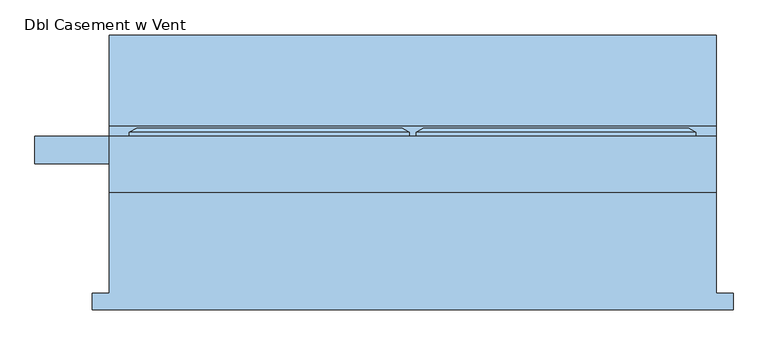
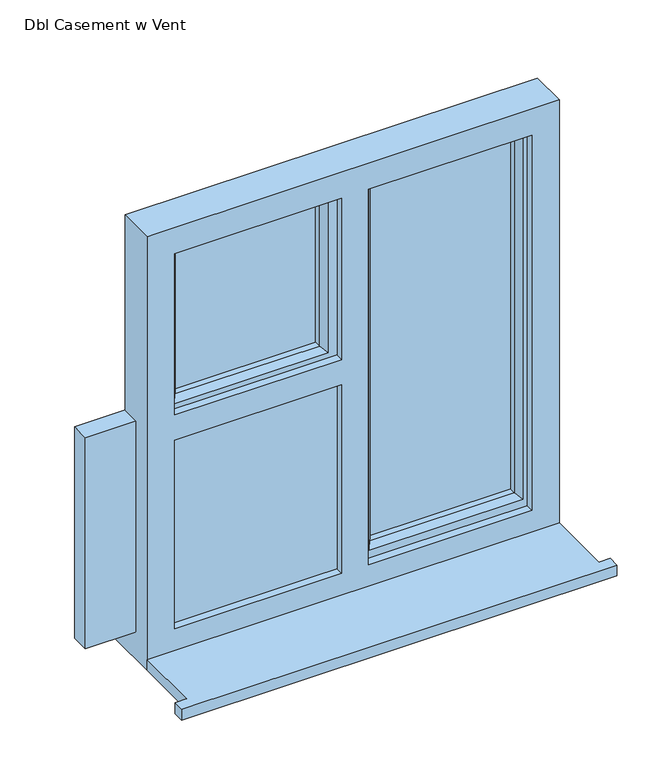
"""IFC4 building model written with IfcOpenShell, lengths in millimetres: window geometry, Dbl Casement w Vent : Doublel Casement with Vent 900w x 1000h."""

import ifcopenshell
import ifcopenshell.guid

model = None  # the IFC model being written
_history = None  # IfcOwnerHistory: only IFC2X3 demands one
_inside = {}  # id of a spatial element -> (the spatial element, [elements in it])
_under = {}  # id of a project, library or spatial element -> (it, [spatial elements below it])
_declared = {}  # id of a project -> (the project, [libraries it declares])
_typed = {}  # id of a type object -> (the type object, [elements of that type])
_made_of = {}  # id of a material, layer set ... -> (it, [elements and type objects made of it])


def new_model(schema):
    """Start an empty IFC model of exactly this schema.

    Asked for "IFC4X3", IfcOpenShell would pick the latest addendum, in which some entities
    have other attributes; the version numbers below select the first issue.
    IFC2X3 requires an IfcOwnerHistory on every rooted entity: one is made here for all.
    """
    global model, _history
    if schema == "IFC4X3":
        model = ifcopenshell.file(schema_version=(4, 3, 0, 0))
    else:
        model = ifcopenshell.file(schema=schema)
    _inside.clear()
    _under.clear()
    _declared.clear()
    _typed.clear()
    _made_of.clear()
    _history = None
    if model.schema == "IFC2X3":
        org = make("IfcOrganization", Name="unknown")
        user = make(
            "IfcPersonAndOrganization",
            ThePerson=make("IfcPerson", FamilyName="unknown"),
            TheOrganization=org,
        )
        app = make(
            "IfcApplication",
            ApplicationDeveloper=org,
            Version="unknown",
            ApplicationFullName="unknown",
            ApplicationIdentifier="unknown",
        )
        _history = make(
            "IfcOwnerHistory",
            OwningUser=user,
            OwningApplication=app,
            ChangeAction="ADDED",
            CreationDate=0,
        )
    return model


def make(cls, **values):
    """One entity of the class cls with the attributes given. An attribute that is None is left unset."""
    return model.create_entity(
        cls, **{name: value for name, value in values.items() if value is not None}
    )


def rooted(cls, **values):
    """An entity with a GlobalId (a new one), such as an element, a storey or a relation."""
    return make(cls, GlobalId=ifcopenshell.guid.new(), OwnerHistory=_history, **values)


def si_unit(unit_type, name, prefix=None):
    """IfcSIUnit, for example si_unit("LENGTHUNIT", "METRE", prefix="MILLI")."""
    return make("IfcSIUnit", UnitType=unit_type, Prefix=prefix, Name=name)


def assignment(units):
    """IfcUnitAssignment: the units of a project."""
    return None if units is None else make("IfcUnitAssignment", Units=units)


def point(xyz):
    """IfcCartesianPoint."""
    return None if xyz is None else make("IfcCartesianPoint", Coordinates=xyz)


def direction(xyz):
    """IfcDirection."""
    return None if xyz is None else make("IfcDirection", DirectionRatios=xyz)


def frame(location, z_axis=None, x_axis=None):
    """IfcAxis2Placement3D, a coordinate frame: its origin and axes. An axis left out is left unset."""
    return make(
        "IfcAxis2Placement3D",
        Location=point(location),
        Axis=direction(z_axis),
        RefDirection=direction(x_axis),
    )


def origin():
    """The frame at (0, 0, 0) with its axes left unset."""
    return frame((0.0, 0.0, 0.0))


def place(relative_to, where):
    """IfcLocalPlacement: puts the frame where relative to a parent placement (None: the world)."""
    return make(
        "IfcLocalPlacement", PlacementRelTo=relative_to, RelativePlacement=where
    )


def context(
    kind, dimensions, precision=None, world=None, true_north=None, identifier=None
):
    """IfcGeometricRepresentationContext, for example the 3D "Model" context."""
    return make(
        "IfcGeometricRepresentationContext",
        ContextIdentifier=identifier,
        ContextType=kind,
        CoordinateSpaceDimension=dimensions,
        Precision=precision,
        WorldCoordinateSystem=world,
        TrueNorth=true_north,
    )


def project(units=None, contexts=None):
    """IfcProject with its units and contexts."""
    return rooted(
        "IfcProject",
        Name="project",
        RepresentationContexts=contexts,
        UnitsInContext=assignment(units),
    )


def spatial(cls, under=None, at=None, **own):
    """A site, building, storey or space (cls), placed at a placement, below another one or the project."""
    s = rooted(cls, ObjectPlacement=at, **own)
    if under is not None:
        _under.setdefault(under.id(), (under, []))[1].append(s)
    return s


def polyline(points):
    """IfcPolyline through the points."""
    return make("IfcPolyline", Points=[point(p) for p in points])


def outline(outer, holes=None, kind="AREA"):
    """IfcArbitraryClosedProfileDef: a profile drawn as a closed curve; with holes, ...WithVoids."""
    if holes is None:
        return make("IfcArbitraryClosedProfileDef", ProfileType=kind, OuterCurve=outer)
    return make(
        "IfcArbitraryProfileDefWithVoids",
        ProfileType=kind,
        OuterCurve=outer,
        InnerCurves=holes,
    )


def extrude(swept, where, along, depth):
    """IfcExtrudedAreaSolid: the profile swept, set in the frame where, extruded along a direction by depth."""
    return make(
        "IfcExtrudedAreaSolid",
        SweptArea=swept,
        Position=where,
        ExtrudedDirection=direction(along),
        Depth=depth,
    )


def faces_of(points, faces, orient=None, outer=None):
    """IfcFace entities. A face is a list of loops; a loop is a list of indices into points, from 0.

    orient and outer hold one flag for each loop. By default every Orientation is true, the
    first loop of a face is its IfcFaceOuterBound and the others are IfcFaceBound.
    """
    made = []
    for i, loops in enumerate(faces):
        bounds = []
        for j, loop in enumerate(loops):
            is_outer = j == 0 if outer is None else outer[i][j]
            bounds.append(
                make(
                    "IfcFaceOuterBound" if is_outer else "IfcFaceBound",
                    Bound=make("IfcPolyLoop", Polygon=[points[k] for k in loop]),
                    Orientation=True if orient is None else orient[i][j],
                )
            )
        made.append(make("IfcFace", Bounds=bounds))
    return made


def faceted_brep(points, faces, orient=None, outer=None, voids=None):
    """IfcFacetedBrep: a solid bounded by flat faces; with voids (closed shells), ...WithVoids."""
    shared = [point(p) for p in points]
    hull = make("IfcClosedShell", CfsFaces=faces_of(shared, faces, orient, outer))
    if voids is None:
        return make("IfcFacetedBrep", Outer=hull)
    return make(
        "IfcFacetedBrepWithVoids",
        Outer=hull,
        Voids=[
            make(cls, CfsFaces=faces_of(shared, fs, o, b)) for cls, fs, o, b in voids
        ],
    )


def shape(context_of_items, identifier, shape_type, items):
    """IfcShapeRepresentation: the items that make up one representation, for example the "Body"."""
    return make(
        "IfcShapeRepresentation",
        ContextOfItems=context_of_items,
        RepresentationIdentifier=identifier,
        RepresentationType=shape_type,
        Items=items,
    )


def source(mapping_origin, context_of_items, identifier, shape_type, items):
    """IfcRepresentationMap: a shape defined once, which mapped items show again and again."""
    return make(
        "IfcRepresentationMap",
        MappingOrigin=mapping_origin,
        MappedRepresentation=shape(context_of_items, identifier, shape_type, items),
    )


def transform(
    local_origin,
    x_axis=None,
    y_axis=None,
    z_axis=None,
    scale=None,
    scale2=None,
    scale3=None,
    uniform=True,
):
    """IfcCartesianTransformationOperator3D, or its non-uniform kind. x_axis, y_axis, z_axis: its Axis1, 2, 3."""
    if uniform:
        return make(
            "IfcCartesianTransformationOperator3D",
            Axis1=direction(x_axis),
            Axis2=direction(y_axis),
            LocalOrigin=point(local_origin),
            Scale=scale,
            Axis3=direction(z_axis),
        )
    return make(
        "IfcCartesianTransformationOperator3DnonUniform",
        Axis1=direction(x_axis),
        Axis2=direction(y_axis),
        LocalOrigin=point(local_origin),
        Scale=scale,
        Axis3=direction(z_axis),
        Scale2=scale2,
        Scale3=scale3,
    )


def mapped(mapping_source, mapping_target):
    """IfcMappedItem: shows the shape of a source again, moved by a transform."""
    return make(
        "IfcMappedItem", MappingSource=mapping_source, MappingTarget=mapping_target
    )


def made_of(thing, what):
    """Note that an element or type object is made of a material, layer set ...; save() writes the relation."""
    if what is not None:
        _made_of.setdefault(what.id(), (what, []))[1].append(thing)
    return thing


def element(
    cls,
    number,
    at=None,
    inside=None,
    cuts=None,
    type_object=None,
    material=None,
    context=None,
    identifier="Body",
    shape_type=None,
    held_by="IfcProductDefinitionShape",
    body=None,
    shapes=None,
    **own,
):
    """One element of the class cls, such as IfcWall. Its Tag is "e" and its number.

    at: its placement. inside: the storey or other place that contains it. cuts: it is an
    opening in that element (IfcRelVoidsElement). A single representation is given by context,
    identifier, shape_type and body (its items); several are given by shapes. held_by: the class
    of the entity that holds the representations. save() writes the other relations.
    """
    e = rooted(cls, Tag="e%d" % number, ObjectPlacement=at, **own)
    if body is not None:
        shapes = [shape(context, identifier, shape_type, body)]
    if shapes is not None:
        e.Representation = make(held_by, Representations=shapes)
    if inside is not None:
        _inside.setdefault(inside.id(), (inside, []))[1].append(e)
    if cuts is not None:
        rooted(
            "IfcRelVoidsElement", RelatingBuildingElement=cuts, RelatedOpeningElement=e
        )
    if type_object is not None:
        _typed.setdefault(type_object.id(), (type_object, []))[1].append(e)
    return made_of(e, material)


def aggregate(whole, parts):
    """IfcRelAggregates: a whole, such as a stair, and the parts it consists of."""
    return rooted("IfcRelAggregates", RelatingObject=whole, RelatedObjects=parts)


def save(model, path):
    """Write the relations noted so far, then the file.

    IfcRelAggregates (storeys below a building ...), IfcRelContainedInSpatialStructure (elements
    in a storey), IfcRelDefinesByType, IfcRelAssociatesMaterial and IfcRelDeclares: one each for
    every whole, place, type object, material and project.
    """
    for whole, parts in _under.values():
        aggregate(whole, parts)
    for where, things in _inside.values():
        rooted(
            "IfcRelContainedInSpatialStructure",
            RelatedElements=things,
            RelatingStructure=where,
        )
    for kind, things in _typed.values():
        rooted("IfcRelDefinesByType", RelatedObjects=things, RelatingType=kind)
    for what, things in _made_of.values():
        rooted("IfcRelAssociatesMaterial", RelatedObjects=things, RelatingMaterial=what)
    for by, libraries in _declared.values():
        rooted("IfcRelDeclares", RelatingContext=by, RelatedDefinitions=libraries)
    model.write(path)


def dbl_casement_w_vent_ca28e73d(model_context):
    return source(origin(), model_context, "Body", "SolidModel", [
        extrude(outline(polyline([(-760.0, -182.7934322), (-760.0, -157.7934322), (-735.0, -157.7934322), (-735.0, -8.2934322), (165.0, -8.2934322), (165.0, -157.7934322), (190.0, -157.7934322), (190.0, -182.7934322), (-760.0, -182.7934322)])), frame((0.0, 0.0, 1110.0), z_axis=(0.0, 0.0, 1.0), x_axis=(1.0, 0.0, 0.0)), (0.0, 0.0, 1.0), 25.0),
        faceted_brep([(-705.0, 74.7065678, 2080.0), (-705.0, 80.4800705, 2080.0), (-705.0, 80.4800705, 1650.0), (-705.0, 74.7065678, 1650.0), (-695.0, 9.7065678, 2070.0), (-695.0, 74.7065678, 2070.0), (-695.0, 74.7065678, 1660.0), (-695.0, 9.7065678, 1660.0), (-655.0, 24.1994677, 2030.0), (-665.1480377, 9.7065678, 2040.1480377), (-665.1480377, 9.7065678, 1689.8519623), (-655.0, 24.1994677, 1700.0), (-655.0, 38.7065678, 2030.0), (-655.0, 38.7065678, 1700.0), (-665.0, 62.7065678, 2040.0), (-665.0, 38.7065678, 2040.0), (-665.0, 38.7065678, 1690.0), (-665.0, 62.7065678, 1690.0), (-655.0, 80.4800705, 2030.0), (-655.0, 62.7065678, 2030.0), (-655.0, 62.7065678, 1700.0), (-655.0, 80.4800705, 1700.0), (-672.4457548, 86.2535732, 2047.4457548), (-672.4457548, 86.2535732, 1682.5542452), (-694.2153903, 86.2535732, 2069.2153903), (-694.2153903, 86.2535732, 1660.7846097), (-290.0, 80.4800705, 1650.0), (-290.0, 74.7065678, 1650.0), (-300.0, 74.7065678, 1660.0), (-300.0, 9.7065678, 1660.0), (-329.8519623, 9.7065678, 1689.8519623), (-340.0, 24.1994677, 1700.0), (-340.0, 38.7065678, 1700.0), (-330.0, 38.7065678, 1690.0), (-330.0, 62.7065678, 1690.0), (-340.0, 62.7065678, 1700.0), (-340.0, 80.4800705, 1700.0), (-322.5542452, 86.2535732, 1682.5542452), (-300.7846097, 86.2535732, 1660.7846097), (-290.0, 80.4800705, 2080.0), (-290.0, 74.7065678, 2080.0), (-300.0, 74.7065678, 2070.0), (-300.0, 9.7065678, 2070.0), (-329.8519623, 9.7065678, 2040.1480377), (-340.0, 24.1994677, 2030.0), (-340.0, 38.7065678, 2030.0), (-330.0, 38.7065678, 2040.0), (-330.0, 62.7065678, 2040.0), (-340.0, 62.7065678, 2030.0), (-340.0, 80.4800705, 2030.0), (-322.5542452, 86.2535732, 2047.4457548), (-300.7846097, 86.2535732, 2069.2153903)], [[[0, 1, 2, 3]], [[4, 5, 6, 7]], [[8, 9, 10, 11]], [[12, 8, 11, 13]], [[14, 15, 16, 17]], [[18, 19, 20, 21]], [[22, 18, 21, 23]], [[1, 24, 25, 2]], [[3, 2, 26, 27]], [[7, 6, 28, 29]], [[11, 10, 30, 31]], [[13, 11, 31, 32]], [[17, 16, 33, 34]], [[21, 20, 35, 36]], [[23, 21, 36, 37]], [[2, 25, 38, 26]], [[27, 26, 39, 40]], [[29, 28, 41, 42]], [[31, 30, 43, 44]], [[32, 31, 44, 45]], [[34, 33, 46, 47]], [[36, 35, 48, 49]], [[37, 36, 49, 50]], [[26, 38, 51, 39]], [[40, 39, 1, 0]], [[3, 27, 40, 0], [5, 41, 28, 6]], [[42, 41, 5, 4]], [[7, 29, 42, 4], [9, 43, 30, 10]], [[44, 43, 9, 8]], [[45, 44, 8, 12]], [[15, 46, 33, 16], [13, 32, 45, 12]], [[47, 46, 15, 14]], [[17, 34, 47, 14], [19, 48, 35, 20]], [[49, 48, 19, 18]], [[50, 49, 18, 22]], [[24, 51, 38, 25], [23, 37, 50, 22]], [[39, 51, 24, 1]]]),
        extrude(outline(polyline([(95.0, 38.7065678), (-240.0, 38.7065678), (-240.0, 62.7065678), (95.0, 62.7065678), (95.0, 38.7065678)])), frame((0.0, 0.0, 1203.0), z_axis=(0.0, 0.0, 1.0), x_axis=(1.0, 0.0, 0.0)), (0.0, 0.0, 1.0), 837.0),
        extrude(outline(polyline([(-330.0, 38.7065678), (-665.0, 38.7065678), (-665.0, 62.7065678), (-330.0, 62.7065678), (-330.0, 38.7065678)])), frame((0.0, 0.0, 1690.0), z_axis=(0.0, 0.0, 1.0), x_axis=(1.0, 0.0, 0.0)), (0.0, 0.0, 1.0), 350.0),
        extrude(outline(polyline([(-695.0, 33.7065678), (-300.0, 33.7065678), (-300.0, 9.7065678), (-695.0, 9.7065678), (-695.0, 33.7065678)])), frame((0.0, 0.0, 1173.0), z_axis=(0.0, 0.0, 1.0), x_axis=(1.0, 0.0, 0.0)), (0.0, 0.0, 1.0), 457.0),
        faceted_brep([(165.0, -8.2934322, 2110.0), (-735.0, -8.2934322, 2110.0), (-735.0, -8.2934322, 1110.0), (165.0, -8.2934322, 1110.0), (-675.0, -8.2934322, 1185.0), (-675.0, -8.2934322, 1620.0), (-310.0, -8.2934322, 1620.0), (-310.0, -8.2934322, 1185.0), (-675.0, -8.2934322, 2050.0), (-310.0, -8.2934322, 2050.0), (-310.0, -8.2934322, 1678.0), (-675.0, -8.2934322, 1678.0), (-252.0, -8.2934322, 2050.0), (105.0, -8.2934322, 2050.0), (105.0, -8.2934322, 1185.0), (-252.0, -8.2934322, 1185.0), (-735.0, 74.7065678, 2110.0), (-735.0, 74.7065678, 1161.0), (-735.0, 89.7065678, 1159.68767), (-735.0, 89.7065678, 1154.7449676), (-735.0, 224.7065678, 1143.8088847), (-735.0, 224.7065678, 1110.0), (165.0, 74.7065678, 2110.0), (165.0, 74.7065678, 1161.0), (-310.0, 74.7065678, 1173.0), (-310.0, 74.7065678, 1620.0), (-695.0, 74.7065678, 1620.0), (-695.0, 74.7065678, 1173.0), (-310.0, 74.7065678, 2070.0), (-695.0, 74.7065678, 2070.0), (-695.0, 74.7065678, 1660.0), (-310.0, 74.7065678, 1660.0), (125.0, 74.7065678, 1173.0), (125.0, 74.7065678, 2070.0), (-270.0, 74.7065678, 2070.0), (-270.0, 74.7065678, 1173.0), (-695.0, 9.7065678, 2070.0), (-695.0, 9.7065678, 1660.0), (-695.0, 9.7065678, 1630.0), (-695.0, 9.7065678, 1173.0), (-695.0, 33.7065678, 1620.0), (-695.0, 33.7065678, 1630.0), (-300.0, 9.7065678, 2070.0), (-300.0, 9.7065678, 1660.0), (-310.0, 9.7065678, 2050.0), (-675.0, 9.7065678, 2050.0), (-675.0, 9.7065678, 1678.0), (-310.0, 9.7065678, 1678.0), (-270.0, 9.7065678, 2070.0), (125.0, 9.7065678, 2070.0), (125.0, 9.7065678, 1173.0), (-270.0, 9.7065678, 1173.0), (105.0, 9.7065678, 2050.0), (-252.0, 9.7065678, 2050.0), (-252.0, 9.7065678, 1185.0), (105.0, 9.7065678, 1185.0), (-300.0, 9.7065678, 1173.0), (-300.0, 9.7065678, 1630.0), (-675.0, 9.7065678, 1185.0), (-310.0, 9.7065678, 1185.0), (-310.0, 9.7065678, 1620.0), (-675.0, 9.7065678, 1620.0), (-310.0, 33.7065678, 2070.0), (-300.0, 33.7065678, 2070.0), (165.0, 224.7065678, 1110.0), (165.0, 224.7065678, 1143.8088847), (165.0, 89.7065678, 1154.7449676), (165.0, 89.7065678, 1159.68767), (-300.0, 33.7065678, 1660.0), (-300.0, 33.7065678, 1630.0), (-300.0, 33.7065678, 1173.0), (-310.0, 33.7065678, 1660.0), (-310.0, 33.7065678, 1173.0), (-310.0, 33.7065678, 1620.0)], [[[0, 1, 2, 3], [4, 5, 6, 7], [8, 9, 10, 11], [12, 13, 14, 15]], [[1, 16, 17, 18, 19, 20, 21, 2]], [[16, 22, 23, 17], [24, 25, 26, 27], [28, 29, 30, 31], [32, 33, 34, 35]], [[29, 36, 37, 30]], [[38, 39, 27, 26, 40, 41]], [[36, 42, 43, 37], [44, 45, 46, 47]], [[48, 49, 50, 51], [52, 53, 54, 55]], [[56, 39, 38, 57], [58, 59, 60, 61]], [[45, 8, 11, 46]], [[4, 58, 61, 5]], [[1, 0, 22, 16]], [[36, 29, 28, 62, 63, 42]], [[33, 49, 48, 34]], [[8, 45, 44, 9]], [[52, 13, 12, 53]], [[22, 0, 3, 64, 65, 66, 67, 23]], [[33, 32, 50, 49]], [[13, 52, 55, 14]], [[43, 42, 63, 68]], [[69, 70, 56, 57]], [[63, 62, 71, 68]], [[72, 70, 69, 41, 40, 73]], [[62, 28, 31, 71]], [[24, 72, 73, 25]], [[35, 34, 48, 51]], [[53, 12, 15, 54]], [[9, 44, 47, 10]], [[59, 7, 6, 60]], [[64, 3, 2, 21]], [[65, 64, 21, 20]], [[66, 65, 20, 19]], [[67, 66, 19, 18]], [[23, 67, 18, 17]], [[24, 27, 39, 56, 70, 72]], [[32, 35, 51, 50]], [[15, 14, 55, 54]], [[59, 58, 4, 7]], [[57, 38, 41, 69]], [[26, 25, 73, 40]], [[31, 30, 37, 43, 68, 71]], [[47, 46, 11, 10]], [[61, 60, 6, 5]]]),
        extrude(outline(polyline([(1660.0, -675.0), (1660.0, -845.0), (1173.0, -845.0), (1173.0, -310.0), (1343.0, -310.0), (1343.0, -675.0), (1660.0, -675.0)])), frame((0.0, 33.7065678, 0.0), z_axis=(0.0, 1.0, 0.0), x_axis=(0.0, 0.0, 1.0)), (0.0, 0.0, 1.0), 41.0),
        faceted_brep([(-280.0, 74.7065678, 2080.0), (-280.0, 80.4800705, 2080.0), (-280.0, 80.4800705, 1163.0), (-280.0, 74.7065678, 1163.0), (-270.0, 9.7065678, 2070.0), (-270.0, 74.7065678, 2070.0), (-270.0, 74.7065678, 1173.0), (-270.0, 9.7065678, 1173.0), (-230.0, 24.1994677, 2030.0), (-240.1480377, 9.7065678, 2040.1480377), (-240.1480377, 9.7065678, 1202.8519623), (-230.0, 24.1994677, 1213.0), (-230.0, 38.7065678, 2030.0), (-230.0, 38.7065678, 1213.0), (-240.0, 62.7065678, 2040.0), (-240.0, 38.7065678, 2040.0), (-240.0, 38.7065678, 1203.0), (-240.0, 62.7065678, 1203.0), (-230.0, 80.4800705, 2030.0), (-230.0, 62.7065678, 2030.0), (-230.0, 62.7065678, 1213.0), (-230.0, 80.4800705, 1213.0), (-247.4457548, 86.2535732, 2047.4457548), (-247.4457548, 86.2535732, 1195.5542452), (-269.2153903, 86.2535732, 2069.2153903), (-269.2153903, 86.2535732, 1173.7846097), (135.0, 80.4800705, 1163.0), (135.0, 74.7065678, 1163.0), (125.0, 74.7065678, 1173.0), (125.0, 9.7065678, 1173.0), (95.1480377, 9.7065678, 1202.8519623), (85.0, 24.1994677, 1213.0), (85.0, 38.7065678, 1213.0), (95.0, 38.7065678, 1203.0), (95.0, 62.7065678, 1203.0), (85.0, 62.7065678, 1213.0), (85.0, 80.4800705, 1213.0), (102.4457548, 86.2535732, 1195.5542452), (124.2153903, 86.2535732, 1173.7846097), (135.0, 80.4800705, 2080.0), (135.0, 74.7065678, 2080.0), (125.0, 74.7065678, 2070.0), (125.0, 9.7065678, 2070.0), (95.1480377, 9.7065678, 2040.1480377), (85.0, 24.1994677, 2030.0), (85.0, 38.7065678, 2030.0), (95.0, 38.7065678, 2040.0), (95.0, 62.7065678, 2040.0), (85.0, 62.7065678, 2030.0), (85.0, 80.4800705, 2030.0), (102.4457548, 86.2535732, 2047.4457548), (124.2153903, 86.2535732, 2069.2153903)], [[[0, 1, 2, 3]], [[4, 5, 6, 7]], [[8, 9, 10, 11]], [[12, 8, 11, 13]], [[14, 15, 16, 17]], [[18, 19, 20, 21]], [[22, 18, 21, 23]], [[1, 24, 25, 2]], [[3, 2, 26, 27]], [[7, 6, 28, 29]], [[11, 10, 30, 31]], [[13, 11, 31, 32]], [[17, 16, 33, 34]], [[21, 20, 35, 36]], [[23, 21, 36, 37]], [[2, 25, 38, 26]], [[27, 26, 39, 40]], [[29, 28, 41, 42]], [[31, 30, 43, 44]], [[32, 31, 44, 45]], [[34, 33, 46, 47]], [[36, 35, 48, 49]], [[37, 36, 49, 50]], [[26, 38, 51, 39]], [[40, 39, 1, 0]], [[3, 27, 40, 0], [5, 41, 28, 6]], [[42, 41, 5, 4]], [[7, 29, 42, 4], [9, 43, 30, 10]], [[44, 43, 9, 8]], [[45, 44, 8, 12]], [[15, 46, 33, 16], [13, 32, 45, 12]], [[47, 46, 15, 14]], [[17, 34, 47, 14], [19, 48, 35, 20]], [[49, 48, 19, 18]], [[50, 49, 18, 22]], [[24, 51, 38, 25], [23, 37, 50, 22]], [[39, 51, 24, 1]]]),
    ])


if __name__ == "__main__":
    model = new_model("IFC4")
    model_context = context("Model", 3, world=origin())
    ifc_project = project(units=[si_unit("LENGTHUNIT", "METRE", prefix="MILLI")], contexts=[model_context])
    site = spatial("IfcSite", under=ifc_project)
    building = spatial("IfcBuilding", under=site)
    placement = place(None, origin())
    dbl_casement_w_vent_shape = dbl_casement_w_vent_ca28e73d(model_context)
    element("IfcWindow", 1, ObjectType="Dbl Casement w Vent : Doublel Casement with Vent 900w x 1000h", at=placement, inside=building, context=model_context, shape_type="MappedRepresentation", body=[
        mapped(dbl_casement_w_vent_shape, transform((0.0, 0.0, 0.0), x_axis=(1.0, 0.0, 0.0), y_axis=(0.0, 1.0, 0.0), z_axis=(0.0, 0.0, 1.0))),
    ])
    save(model, "model.ifc")

# Revit data of these elements
# Type "Dbl Casement w Vent : Doublel Casement with Vent 900w x 1000h"
#   Description = "Double Casement Window with Opening Sash Vents"
#   Type Mark = "73"
#   Operation = "TriplePanelRight"
#   Construction Type Id = "GSP4R"
#   Manufacturer = "Revit"
#   Keynote = "L10"
#   Analytic Construction = "1/8 in Pilkington single glazing"
#   Wrap Layers (Ext) from Ext = 102.5 mm
#   Wrap Layers (Int) from Ext = 177.5 mm
#   Window Board Projection = 25 mm
#   Window Board Extension = 25 mm
#   Visual Light Transmittance = 0.9
#   Vent Depth = 450 mm
#   Thermal Resistance (R) = 0.271106 (m²·K)/W
#   Solar Heat Gain Coefficient = 0.78
#   Rough Width = 900 mm
#   Rough Height = 1000 mm
#   Frame Height = 1350 mm
#   Height = 1000 mm
#   Width = 900 mm
#   Heat Transfer Coefficient (U) = 3.6886 W/(m²·K)
#   Glazing Thickness = 24 mm
#   FrameOffset - External = 100 mm
#   Frame Depth = 65 mm
#   Default Head Height = 2110 mm
#   Cill Depth = 150 mm
#   Cavity Closer Width = 75 mm
#   Cavity Closer Offset from Ext = 110 mm
#   Cavity Closer Depth = 105 mm
#   Vis - Cavity Closers = yes
#   Define Thermal Properties by = 1
#   Material Trim = Window Frame
#   Material Glass = Glass
#   Material Frame = Window Frame
#   Wall Closure = (empty or 0)
# Element 1 (IfcWindow, "Dbl Casement w Vent : Doublel Casement with Vent 900w x 1000h")
#   Materials on its faces: "Window Frame", "Glass"
# Materials
#   "Window Frame": class "Miscellaneous", colour RGB 249 249 249, transparency 0, Keynote = "L10"
#   "Glass": class "Glass", colour RGB 0 128 192, transparency 0.9, Description = "Soda Lime Glass", Cost = 0
